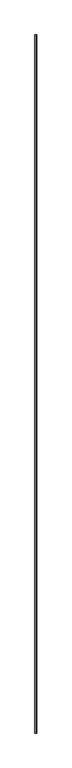
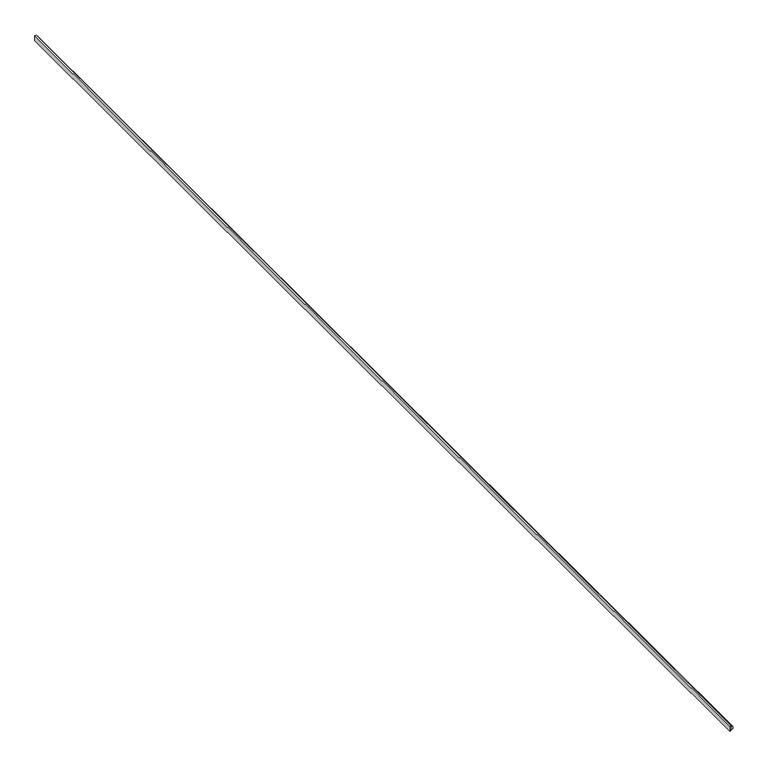
"""IFC4 building model written with IfcOpenShell, lengths in millimetres: proxy geometry, Door frame5:Door frame005:296182 : Door frame5:Door frame005:296182."""

from ifc_helpers import new_model, si_unit, frame, origin, place, context, project, spatial, polyline, outline, extrude, source, transform, mapped, element, save


def generic_models_32f94e88(model_context):
    return source(origin(), model_context, "Body", "SweptSolid", [
        extrude(outline(polyline([(36687.4772673, 20332.3383326), (36678.7014343, 20332.3383326), (36678.7014343, 20334.5557056), (36682.2000947, 20334.5557056), (36682.2000947, 20336.3337056), (36680.8030947, 20336.3337056), (36680.8030947, 20337.4005056), (36685.3750947, 20337.4005056), (36685.3750947, 20336.3337056), (36683.9780947, 20336.3337056), (36683.9780947, 20334.555655), (36687.4772673, 20334.555655), (36687.4772673, 20332.3383326)])), frame((0.0, -774.5581156, 0.0), z_axis=(0.0, 1.0, 0.0), x_axis=(0.0, 0.0, 1.0)), (0.0, 0.0, 1.0), 1999.85),
    ])


if __name__ == "__main__":
    model = new_model("IFC4")
    model_context = context("Model", 3, world=origin())
    ifc_project = project(units=[si_unit("LENGTHUNIT", "METRE", prefix="MILLI")], contexts=[model_context])
    site = spatial("IfcSite", under=ifc_project)
    building = spatial("IfcBuilding", under=site)
    placement = place(None, origin())
    generic_models_shape = generic_models_32f94e88(model_context)
    element("IfcBuildingElementProxy", 1, Name="Door frame5:Door frame005:296182 : Door frame5:Door frame005:296182", ObjectType="Door frame5:Door frame005:296182 : Door frame5:Door frame005:296182", at=placement, inside=building, context=model_context, shape_type="MappedRepresentation", body=[
        mapped(generic_models_shape, transform((0.0, 0.0, 0.0), x_axis=(1.0, 0.0, 0.0), y_axis=(0.0, 1.0, 0.0), z_axis=(0.0, 0.0, 1.0))),
    ])
    save(model, "model.ifc")

# Revit data of these elements
# Type "Door frame5:Door frame005:296182 : Door frame5:Door frame005:296182"
#   NameOverride = "Door frame5:Door frame005:296182"
#   ObjectTypeOverride = "Door frame5:Door frame005"
#   Reference = "Door frame005"
#   Category = "Generic Models"
#   Tag = "296182"
# Element 1 (IfcBuildingElementProxy, "Door frame5:Door frame005:296182 : Door frame5:Door frame005:296182")
#   Materials on its faces: "FLEETWOOD SERIES T-3200 SINGLE SWING DOOR FRAME"
# Materials
#   "FLEETWOOD SERIES T-3200 SINGLE SWING DOOR FRAME": class "Unassigned", colour RGB 128 128 128, transparency 0, Cost = 0
